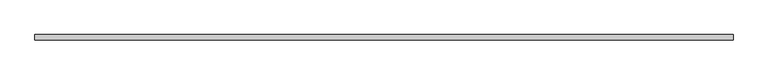
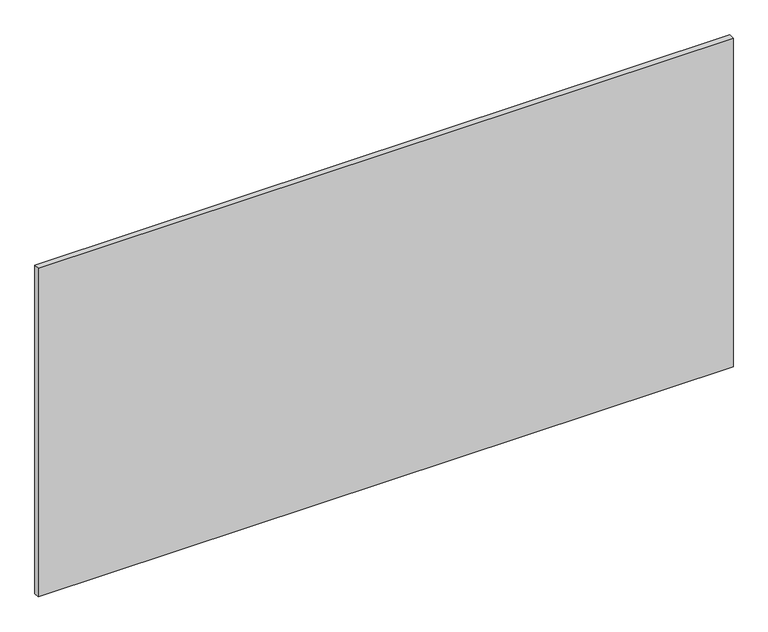
"""IFC4 building model written with IfcOpenShell, lengths in millimetres: proxy geometry, Inner panel:Inner panel:1:Inner panel:1 : Inner panel:Inner panel:300324:300043:Inner panel:1:Inner panel:1 : Inner panel:Inner panel:300324:300043 : Inner panel:Inner panel:1:Inner panel:1 : Inner panel:Inner panel:300324:300043:26 : Inner panel:Inner panel:1:Inner panel:1 : Inner panel:Inner panel:300324:300043:Inner panel:1:Inner panel:1 : Inner panel:Inner panel:300324:300043 : Inner panel:Inner panel:1:Inner panel:1 : Inner panel:Inner panel:300324:300043:300031."""

from ifc_helpers import new_model, si_unit, frame, origin, place, context, project, spatial, polyline, outline, extrude, source, transform, mapped, element, save


def generic_models_3256cd0e(model_context):
    return source(origin(), model_context, "Body", "SweptSolid", [
        extrude(outline(polyline([(590067.7867239, -567913.5913841), (592506.1867239, -567913.5913841), (592506.1867239, -567932.6413841), (590067.7867239, -567932.6413841), (590067.7867239, -567913.5913841)])), frame((0.0, 0.0, 3721.1), z_axis=(0.0, 0.0, 1.0), x_axis=(1.0, 0.0, 0.0)), (0.0, 0.0, 1.0), 1219.2),
    ])


if __name__ == "__main__":
    model = new_model("IFC4")
    model_context = context("Model", 3, world=origin())
    ifc_project = project(units=[si_unit("LENGTHUNIT", "METRE", prefix="MILLI")], contexts=[model_context])
    site = spatial("IfcSite", under=ifc_project)
    building = spatial("IfcBuilding", under=site)
    placement = place(None, origin())
    generic_models_shape = generic_models_3256cd0e(model_context)
    element("IfcBuildingElementProxy", 1, Name="Inner panel:Inner panel:1:Inner panel:1 : Inner panel:Inner panel:300324:300043:Inner panel:1:Inner panel:1 : Inner panel:Inner panel:300324:300043 : Inner panel:Inner panel:1:Inner panel:1 : Inner panel:Inner panel:300324:300043:26 : Inner panel:Inner panel:1:Inner panel:1 : Inner panel:Inner panel:300324:300043:Inner panel:1:Inner panel:1 : Inner panel:Inner panel:300324:300043 : Inner panel:Inner panel:1:Inner panel:1 : Inner panel:Inner panel:300324:300043:300031", ObjectType="Inner panel:Inner panel:1:Inner panel:1 : Inner panel:Inner panel:300324:300043:Inner panel:1:Inner panel:1 : Inner panel:Inner panel:300324:300043 : Inner panel:Inner panel:1:Inner panel:1 : Inner panel:Inner panel:300324:300043:26 : Inner panel:Inner panel:1:Inner panel:1 : Inner panel:Inner panel:300324:300043:Inner panel:1:Inner panel:1 : Inner panel:Inner panel:300324:300043 : Inner panel:Inner panel:1:Inner panel:1 : Inner panel:Inner panel:300324:300043:300031", at=placement, inside=building, context=model_context, shape_type="MappedRepresentation", body=[
        mapped(generic_models_shape, transform((0.0, 0.0, 0.0), x_axis=(1.0, 0.0, 0.0), y_axis=(0.0, 1.0, 0.0), z_axis=(0.0, 0.0, 1.0))),
    ])
    save(model, "model.ifc")

# Revit data of these elements
# Type "Inner panel:Inner panel:1:Inner panel:1 : Inner panel:Inner panel:300324:300043:Inner panel:1:Inner panel:1 : Inner panel:Inner panel:300324:300043 : Inner panel:Inner panel:1:Inner panel:1 : Inner panel:Inner panel:300324:300043:26 : Inner panel:Inner panel:1:Inner panel:1 : Inner panel:Inner panel:300324:300043:Inner panel:1:Inner panel:1 : Inner panel:Inner panel:300324:300043 : Inner panel:Inner panel:1:Inner panel:1 : Inner panel:Inner panel:300324:300043:300031"
#   NameOverride = "Inner panel:Inner panel:1:Inner panel:1 : Inner panel:Inner panel:300324:300043:Inner panel:1:Inner panel:1 : Inner panel:Inner panel:300324:300043 : Inner panel:Inner panel:1:Inner panel:1 : Inner panel:Inner panel:300324:300043:300031"
#   ObjectTypeOverride = "Inner panel:1:Inner panel:1 : Inner panel:Inner panel:300324:300043 : Inner panel:Inner panel:1:Inner panel:1 : Inner panel:Inner panel:300324:300043"
#   Reference = "Inner panel"
#   Tag = "300031"
# Element 1 (IfcBuildingElementProxy, "Inner panel:Inner panel:1:Inner panel:1 : Inner panel:Inner panel:300324:300043:Inner panel:1:Inner panel:1 : Inner panel:Inner panel:300324:300043 : Inner panel:Inner panel:1:Inner panel:1 : Inner panel:Inner panel:300324:300043:26 : Inner panel:Inner panel:1:Inner panel:1 : Inner panel:Inner panel:300324:300043:Inner panel:1:Inner panel:1 : Inner panel:Inner panel:300324:300043 : Inner panel:Inner panel:1:Inner panel:1 : Inner panel:Inner panel:300324:300043:300031")
#   Materials on its faces: "¾” (CLASS A) FIRE RETARDANT PLYWOOD ...OR… IF 1/4\" GYP. BD UNDER PLYWOOD, FLAME SPREAD TO BE CLASS C -  (FINISH: GRADE B - PREFINISHED STAINED/SEALED) - 1/4\" GAP BTWN PANELS (FASTENERS T.B.D.)"
# Materials
#   "¾” (CLASS A) FIRE RETARDANT PLYWOOD ...OR… IF 1/4\" GYP. BD UNDER PLYWOOD, FLAME SPREAD TO BE CLASS C -  (FINISH: GRADE B - PREFINISHED STAINED/SEALED) - 1/4\" GAP BTWN PANELS (FASTENERS T.B.D.)": class "Wood", colour RGB 149 120 74, transparency 0, Description = "Plywood, sheathing grade", Cost = 0
